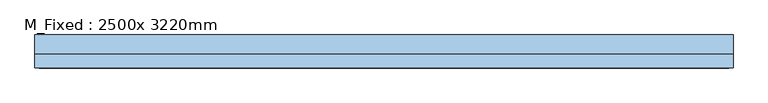
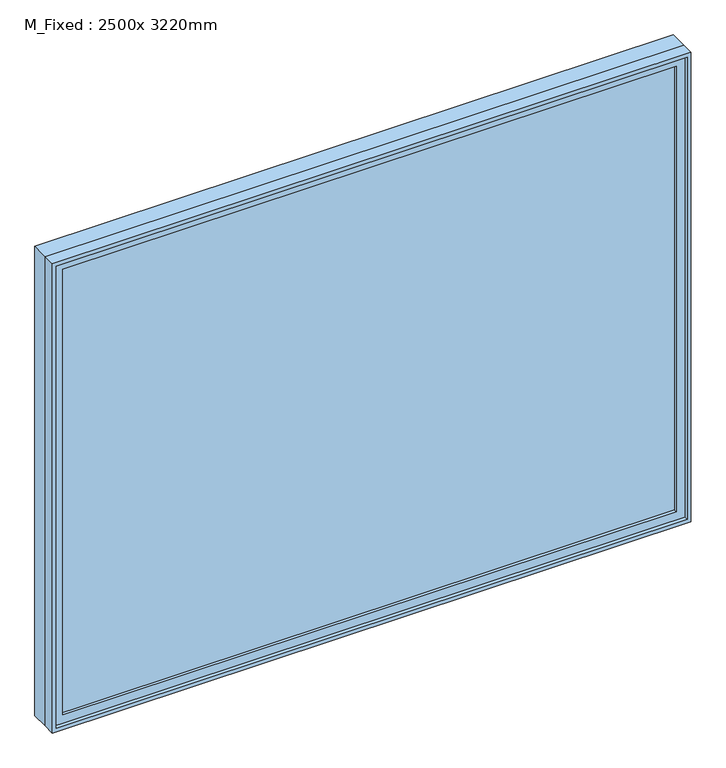
"""IFC4 building model written with IfcOpenShell, lengths in millimetres: window geometry, M_Fixed : 2500x 3220mm."""

import ifcopenshell
import ifcopenshell.guid

model = None  # the IFC model being written
_history = None  # IfcOwnerHistory: only IFC2X3 demands one
_inside = {}  # id of a spatial element -> (the spatial element, [elements in it])
_under = {}  # id of a project, library or spatial element -> (it, [spatial elements below it])
_declared = {}  # id of a project -> (the project, [libraries it declares])
_typed = {}  # id of a type object -> (the type object, [elements of that type])
_made_of = {}  # id of a material, layer set ... -> (it, [elements and type objects made of it])


def new_model(schema):
    """Start an empty IFC model of exactly this schema.

    Asked for "IFC4X3", IfcOpenShell would pick the latest addendum, in which some entities
    have other attributes; the version numbers below select the first issue.
    IFC2X3 requires an IfcOwnerHistory on every rooted entity: one is made here for all.
    """
    global model, _history
    if schema == "IFC4X3":
        model = ifcopenshell.file(schema_version=(4, 3, 0, 0))
    else:
        model = ifcopenshell.file(schema=schema)
    _inside.clear()
    _under.clear()
    _declared.clear()
    _typed.clear()
    _made_of.clear()
    _history = None
    if model.schema == "IFC2X3":
        org = make("IfcOrganization", Name="unknown")
        user = make(
            "IfcPersonAndOrganization",
            ThePerson=make("IfcPerson", FamilyName="unknown"),
            TheOrganization=org,
        )
        app = make(
            "IfcApplication",
            ApplicationDeveloper=org,
            Version="unknown",
            ApplicationFullName="unknown",
            ApplicationIdentifier="unknown",
        )
        _history = make(
            "IfcOwnerHistory",
            OwningUser=user,
            OwningApplication=app,
            ChangeAction="ADDED",
            CreationDate=0,
        )
    return model


def make(cls, **values):
    """One entity of the class cls with the attributes given. An attribute that is None is left unset."""
    return model.create_entity(
        cls, **{name: value for name, value in values.items() if value is not None}
    )


def rooted(cls, **values):
    """An entity with a GlobalId (a new one), such as an element, a storey or a relation."""
    return make(cls, GlobalId=ifcopenshell.guid.new(), OwnerHistory=_history, **values)


def si_unit(unit_type, name, prefix=None):
    """IfcSIUnit, for example si_unit("LENGTHUNIT", "METRE", prefix="MILLI")."""
    return make("IfcSIUnit", UnitType=unit_type, Prefix=prefix, Name=name)


def assignment(units):
    """IfcUnitAssignment: the units of a project."""
    return None if units is None else make("IfcUnitAssignment", Units=units)


def point(xyz):
    """IfcCartesianPoint."""
    return None if xyz is None else make("IfcCartesianPoint", Coordinates=xyz)


def direction(xyz):
    """IfcDirection."""
    return None if xyz is None else make("IfcDirection", DirectionRatios=xyz)


def frame(location, z_axis=None, x_axis=None):
    """IfcAxis2Placement3D, a coordinate frame: its origin and axes. An axis left out is left unset."""
    return make(
        "IfcAxis2Placement3D",
        Location=point(location),
        Axis=direction(z_axis),
        RefDirection=direction(x_axis),
    )


def origin():
    """The frame at (0, 0, 0) with its axes left unset."""
    return frame((0.0, 0.0, 0.0))


def place(relative_to, where):
    """IfcLocalPlacement: puts the frame where relative to a parent placement (None: the world)."""
    return make(
        "IfcLocalPlacement", PlacementRelTo=relative_to, RelativePlacement=where
    )


def context(
    kind, dimensions, precision=None, world=None, true_north=None, identifier=None
):
    """IfcGeometricRepresentationContext, for example the 3D "Model" context."""
    return make(
        "IfcGeometricRepresentationContext",
        ContextIdentifier=identifier,
        ContextType=kind,
        CoordinateSpaceDimension=dimensions,
        Precision=precision,
        WorldCoordinateSystem=world,
        TrueNorth=true_north,
    )


def project(units=None, contexts=None):
    """IfcProject with its units and contexts."""
    return rooted(
        "IfcProject",
        Name="project",
        RepresentationContexts=contexts,
        UnitsInContext=assignment(units),
    )


def spatial(cls, under=None, at=None, **own):
    """A site, building, storey or space (cls), placed at a placement, below another one or the project."""
    s = rooted(cls, ObjectPlacement=at, **own)
    if under is not None:
        _under.setdefault(under.id(), (under, []))[1].append(s)
    return s


def polyline(points):
    """IfcPolyline through the points."""
    return make("IfcPolyline", Points=[point(p) for p in points])


def outline(outer, holes=None, kind="AREA"):
    """IfcArbitraryClosedProfileDef: a profile drawn as a closed curve; with holes, ...WithVoids."""
    if holes is None:
        return make("IfcArbitraryClosedProfileDef", ProfileType=kind, OuterCurve=outer)
    return make(
        "IfcArbitraryProfileDefWithVoids",
        ProfileType=kind,
        OuterCurve=outer,
        InnerCurves=holes,
    )


def extrude(swept, where, along, depth):
    """IfcExtrudedAreaSolid: the profile swept, set in the frame where, extruded along a direction by depth."""
    return make(
        "IfcExtrudedAreaSolid",
        SweptArea=swept,
        Position=where,
        ExtrudedDirection=direction(along),
        Depth=depth,
    )


def shape(context_of_items, identifier, shape_type, items):
    """IfcShapeRepresentation: the items that make up one representation, for example the "Body"."""
    return make(
        "IfcShapeRepresentation",
        ContextOfItems=context_of_items,
        RepresentationIdentifier=identifier,
        RepresentationType=shape_type,
        Items=items,
    )


def source(mapping_origin, context_of_items, identifier, shape_type, items):
    """IfcRepresentationMap: a shape defined once, which mapped items show again and again."""
    return make(
        "IfcRepresentationMap",
        MappingOrigin=mapping_origin,
        MappedRepresentation=shape(context_of_items, identifier, shape_type, items),
    )


def transform(
    local_origin,
    x_axis=None,
    y_axis=None,
    z_axis=None,
    scale=None,
    scale2=None,
    scale3=None,
    uniform=True,
):
    """IfcCartesianTransformationOperator3D, or its non-uniform kind. x_axis, y_axis, z_axis: its Axis1, 2, 3."""
    if uniform:
        return make(
            "IfcCartesianTransformationOperator3D",
            Axis1=direction(x_axis),
            Axis2=direction(y_axis),
            LocalOrigin=point(local_origin),
            Scale=scale,
            Axis3=direction(z_axis),
        )
    return make(
        "IfcCartesianTransformationOperator3DnonUniform",
        Axis1=direction(x_axis),
        Axis2=direction(y_axis),
        LocalOrigin=point(local_origin),
        Scale=scale,
        Axis3=direction(z_axis),
        Scale2=scale2,
        Scale3=scale3,
    )


def mapped(mapping_source, mapping_target):
    """IfcMappedItem: shows the shape of a source again, moved by a transform."""
    return make(
        "IfcMappedItem", MappingSource=mapping_source, MappingTarget=mapping_target
    )


def made_of(thing, what):
    """Note that an element or type object is made of a material, layer set ...; save() writes the relation."""
    if what is not None:
        _made_of.setdefault(what.id(), (what, []))[1].append(thing)
    return thing


def element(
    cls,
    number,
    at=None,
    inside=None,
    cuts=None,
    type_object=None,
    material=None,
    context=None,
    identifier="Body",
    shape_type=None,
    held_by="IfcProductDefinitionShape",
    body=None,
    shapes=None,
    **own,
):
    """One element of the class cls, such as IfcWall. Its Tag is "e" and its number.

    at: its placement. inside: the storey or other place that contains it. cuts: it is an
    opening in that element (IfcRelVoidsElement). A single representation is given by context,
    identifier, shape_type and body (its items); several are given by shapes. held_by: the class
    of the entity that holds the representations. save() writes the other relations.
    """
    e = rooted(cls, Tag="e%d" % number, ObjectPlacement=at, **own)
    if body is not None:
        shapes = [shape(context, identifier, shape_type, body)]
    if shapes is not None:
        e.Representation = make(held_by, Representations=shapes)
    if inside is not None:
        _inside.setdefault(inside.id(), (inside, []))[1].append(e)
    if cuts is not None:
        rooted(
            "IfcRelVoidsElement", RelatingBuildingElement=cuts, RelatedOpeningElement=e
        )
    if type_object is not None:
        _typed.setdefault(type_object.id(), (type_object, []))[1].append(e)
    return made_of(e, material)


def aggregate(whole, parts):
    """IfcRelAggregates: a whole, such as a stair, and the parts it consists of."""
    return rooted("IfcRelAggregates", RelatingObject=whole, RelatedObjects=parts)


def save(model, path):
    """Write the relations noted so far, then the file.

    IfcRelAggregates (storeys below a building ...), IfcRelContainedInSpatialStructure (elements
    in a storey), IfcRelDefinesByType, IfcRelAssociatesMaterial and IfcRelDeclares: one each for
    every whole, place, type object, material and project.
    """
    for whole, parts in _under.values():
        aggregate(whole, parts)
    for where, things in _inside.values():
        rooted(
            "IfcRelContainedInSpatialStructure",
            RelatedElements=things,
            RelatingStructure=where,
        )
    for kind, things in _typed.values():
        rooted("IfcRelDefinesByType", RelatedObjects=things, RelatingType=kind)
    for what, things in _made_of.values():
        rooted("IfcRelAssociatesMaterial", RelatedObjects=things, RelatingMaterial=what)
    for by, libraries in _declared.values():
        rooted("IfcRelDeclares", RelatingContext=by, RelatedDefinitions=libraries)
    model.write(path)


def m_fixed_2500x_3220mm_8b997f8c(model_context):
    return source(origin(), model_context, "Body", "SweptSolid", [
        extrude(outline(polyline([(-1546.8, -54.2), (-1546.8, -42.2), (1546.8, -42.2), (1546.8, -54.2), (-1546.8, -54.2)])), frame((0.0, 0.0, 368.0), z_axis=(0.0, 0.0, 1.0), x_axis=(1.0, 0.0, 0.0)), (0.0, 0.0, 1.0), 2374.0),
        extrude(outline(polyline([(2786.0, -1590.8), (324.0, -1590.8), (324.0, 1590.8), (2786.0, 1590.8), (2786.0, -1590.8)]), holes=[polyline([(2742.0, -1546.8), (2742.0, 1546.8), (368.0, 1546.8), (368.0, -1546.8), (2742.0, -1546.8)])]), frame((0.0, -70.2, 0.0), z_axis=(0.0, 1.0, 0.0), x_axis=(0.0, 0.0, 1.0)), (0.0, 0.0, 1.0), 44.0),
        extrude(outline(polyline([(2805.0, -1609.8), (305.0, -1609.8), (305.0, 1609.8), (2805.0, 1609.8), (2805.0, -1609.8)]), holes=[polyline([(2786.0, -1590.8), (2786.0, 1590.8), (324.0, 1590.8), (324.0, -1590.8), (2786.0, -1590.8)])]), frame((0.0, -89.2, 0.0), z_axis=(0.0, 1.0, 0.0), x_axis=(0.0, 0.0, 1.0)), (0.0, 0.0, 1.0), 63.0),
        extrude(outline(polyline([(2805.0, -1609.8), (305.0, -1609.8), (305.0, 1609.8), (2805.0, 1609.8), (2805.0, -1609.8)]), holes=[polyline([(2773.0, -1577.8), (2773.0, 1577.8), (337.0, 1577.8), (337.0, -1577.8), (2773.0, -1577.8)])]), frame((0.0, -26.2, 0.0), z_axis=(0.0, 1.0, 0.0), x_axis=(0.0, 0.0, 1.0)), (0.0, 0.0, 1.0), 89.4),
    ])


if __name__ == "__main__":
    model = new_model("IFC4")
    model_context = context("Model", 3, world=origin())
    ifc_project = project(units=[si_unit("LENGTHUNIT", "METRE", prefix="MILLI")], contexts=[model_context])
    site = spatial("IfcSite", under=ifc_project)
    building = spatial("IfcBuilding", under=site)
    placement = place(None, origin())
    m_fixed_2500x_3220mm_shape = m_fixed_2500x_3220mm_8b997f8c(model_context)
    element("IfcWindow", 1, ObjectType="M_Fixed : 2500x 3220mm", at=placement, inside=building, context=model_context, shape_type="MappedRepresentation", body=[
        mapped(m_fixed_2500x_3220mm_shape, transform((0.0, 0.0, 0.0), x_axis=(1.0, 0.0, 0.0), y_axis=(0.0, 1.0, 0.0), z_axis=(0.0, 0.0, 1.0))),
    ])
    save(model, "model.ifc")

# Revit data of these elements
# Type "M_Fixed : 2500x 3220mm"
#   Type Mark = "26"
#   Height = 2500 mm
#   Default Sill Height = 305 mm
#   Width = 3219.6 mm
#   Window Inset = 19 mm
#   Frame Exterior Material = Sash
#   Frame Interior Material = Sash
#   Glass Pane Material = Glass
#   Sash = Sash
#   Wall Closure = (empty or 0)
# Element 1 (IfcWindow, "M_Fixed : 2500x 3220mm")
#   Materials on its faces: "Sash", "Glass"
# Materials
#   "Sash": class "Wood", colour RGB 136 99 55, transparency 0
#   "Glass": class "Glass", colour RGB 0 128 192, transparency 0.9, Description = "Soda Lime Glass", Cost = 0
